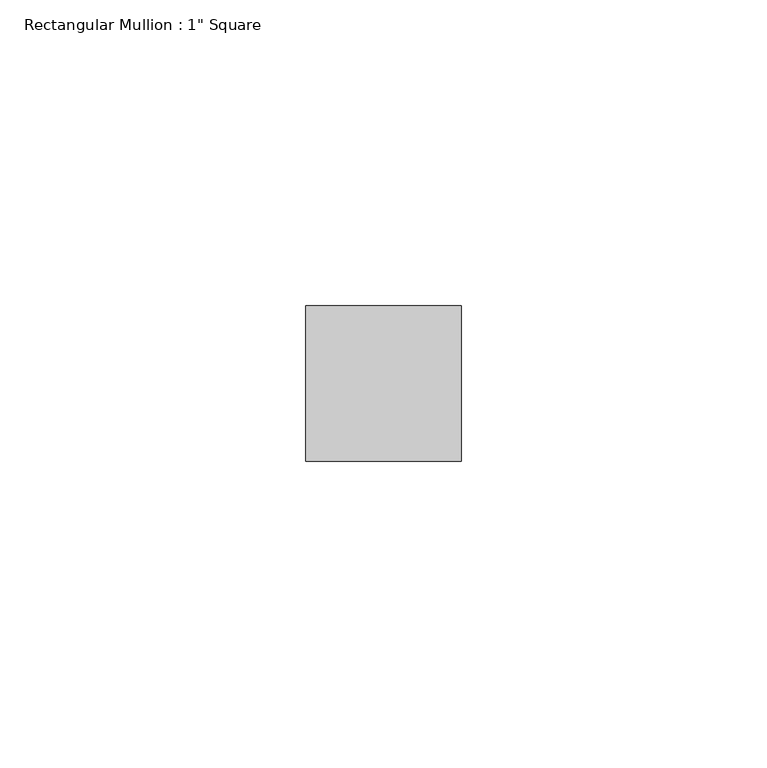
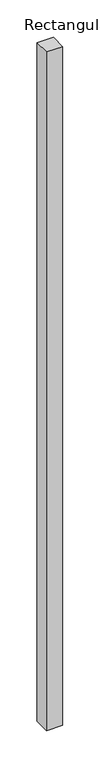
"""IFC4 building model written with IfcOpenShell, lengths in millimetres: member geometry."""

from ifc_helpers import new_model, si_unit, frame, origin, place, context, project, spatial, polyline, outline, extrude, source, transform, mapped, element, save


def member_7d29e2ff(model_context):
    return source(origin(), model_context, "Body", "SweptSolid", [
        extrude(outline(polyline([(0.0, 12.7), (0.0, -12.7), (-25.4, -12.7), (-25.4, 12.7), (0.0, 12.7)])), frame((0.0, 0.0, -1115.149828), z_axis=(0.0, 0.0, 1.0), x_axis=(1.0, 0.0, 0.0)), (0.0, 0.0, 1.0), 1115.149828),
    ])


if __name__ == "__main__":
    model = new_model("IFC4")
    model_context = context("Model", 3, world=origin())
    ifc_project = project(units=[si_unit("LENGTHUNIT", "METRE", prefix="MILLI")], contexts=[model_context])
    site = spatial("IfcSite", under=ifc_project)
    building = spatial("IfcBuilding", under=site)
    placement = place(None, origin())
    member_shape = member_7d29e2ff(model_context)
    element("IfcMember", 1, ObjectType="Rectangular Mullion : 1\" Square", at=placement, inside=building, context=model_context, shape_type="MappedRepresentation", body=[
        mapped(member_shape, transform((0.0, 0.0, 0.0), x_axis=(1.0, 0.0, 0.0), y_axis=(0.0, 1.0, 0.0), z_axis=(0.0, 0.0, 1.0))),
    ])
    save(model, "model.ifc")

# Revit data of these elements
# Type "Rectangular Mullion : 1\" Square"
#   built-in parameter 1007304 = 0.0833333 (stored number, unit not read)
#   built-in parameter 1007301 = 0.0416667 (stored number, unit not read)
#   built-in parameter 1007300 = 0.0416667 (stored number, unit not read)
# Element 1 (IfcMember, "Rectangular Mullion : 1\" Square")
#   Materials on its faces: "Metal - Aluminum"
# Materials
#   "Metal - Aluminum": class "Metal", colour RGB 247 247 247, transparency 0
